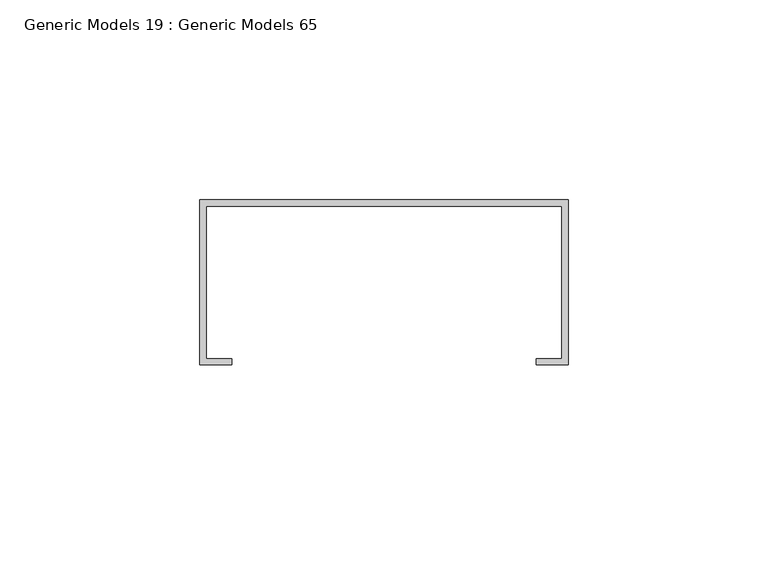
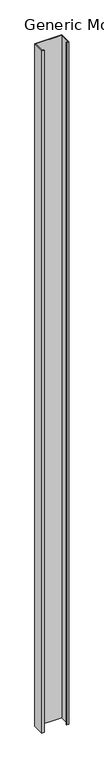
"""IFC4 building model written with IfcOpenShell, lengths in millimetres: proxy geometry, Generic Models 19 : Generic Models 65."""

from ifc_helpers import new_model, si_unit, frame, origin, place, context, project, spatial, polyline, outline, extrude, source, transform, mapped, element, save


def generic_models_19_generic_models_65_4a0df7f0(model_context):
    return source(origin(), model_context, "Body", "SweptSolid", [
        extrude(outline(polyline([(49691.925, 630.2375), (49784.0, 630.2375), (49784.0, 588.9625), (49776.0625, 588.9625), (49776.0625, 590.55), (49782.4125, 590.55), (49782.4125, 628.65), (49693.5125, 628.65), (49693.5125, 590.55), (49699.8625, 590.55), (49699.8625, 588.9625), (49691.925, 588.9625), (49691.925, 630.2375)])), frame((0.0, 0.0, 1.5875), z_axis=(0.0, 0.0, 1.0), x_axis=(1.0, 0.0, 0.0)), (0.0, 0.0, 1.0), 2454.275),
    ])


if __name__ == "__main__":
    model = new_model("IFC4")
    model_context = context("Model", 3, world=origin())
    ifc_project = project(units=[si_unit("LENGTHUNIT", "METRE", prefix="MILLI")], contexts=[model_context])
    site = spatial("IfcSite", under=ifc_project)
    building = spatial("IfcBuilding", under=site)
    placement = place(None, origin())
    generic_models_19_generic_models_65_shape = generic_models_19_generic_models_65_4a0df7f0(model_context)
    element("IfcBuildingElementProxy", 1, Name="Generic Models 19 : Generic Models 65", ObjectType="Generic Models 19 : Generic Models 65", at=placement, inside=building, context=model_context, shape_type="MappedRepresentation", body=[
        mapped(generic_models_19_generic_models_65_shape, transform((0.0, 0.0, 0.0), x_axis=(1.0, 0.0, 0.0), y_axis=(0.0, 1.0, 0.0), z_axis=(0.0, 0.0, 1.0))),
    ])
    save(model, "model.ifc")

# Revit data of these elements
# Element 1 (IfcBuildingElementProxy, "Generic Models 19 : Generic Models 65")
#   Materials on its faces: "METAL STUDS - SEE 'WALL TAG' & 'LAYER MATERIAL SCHEDULE' FOR GAUGE/SPACING & INSULATION TREATMENT, IF APPLICABLE"
# Materials
#   "METAL STUDS - SEE 'WALL TAG' & 'LAYER MATERIAL SCHEDULE' FOR GAUGE/SPACING & INSULATION TREATMENT, IF APPLICABLE": class "Unassigned", colour RGB 210 209 208, transparency 0, Keynote = "M05121300.02", Cost = 0
